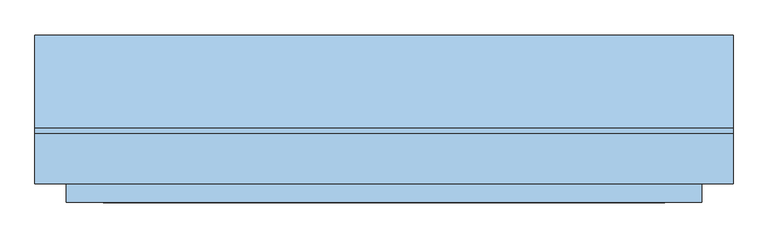
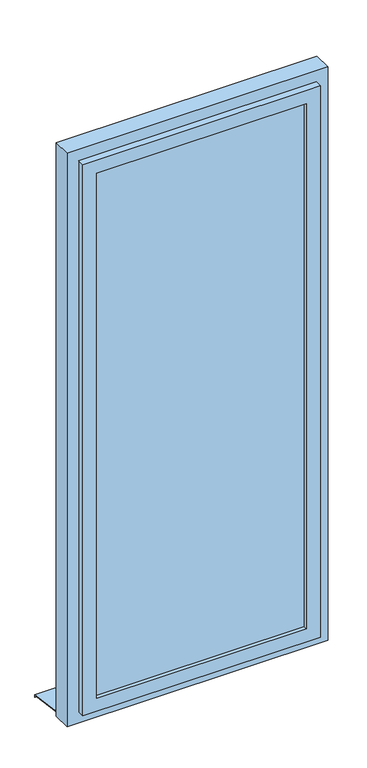
"""IFC4 building model written with IfcOpenShell, lengths in millimetres: window geometry, Fenstertür 1-flg : 1.80 x  3,1."""

from ifc_helpers import new_model, si_unit, frame, origin, place, context, project, spatial, polyline, outline, extrude, faceted_brep, source, transform, mapped, element, save


def window_6dc6708e(model_context):
    return source(origin(), model_context, "Body", "SolidModel", [
        extrude(outline(polyline([(2600.0, 560.0), (2600.0, -560.0), (0.0, -560.0), (0.0, 560.0), (2600.0, 560.0)]), holes=[polyline([(2520.0, 480.0), (80.0, 480.0), (80.0, -480.0), (2520.0, -480.0), (2520.0, 480.0)])]), frame((0.0, -58.6893832, 0.0), z_axis=(0.0, 1.0, 0.0), x_axis=(0.0, 0.0, 1.0)), (0.0, 0.0, 1.0), 80.0),
        faceted_brep([(510.0, -58.6893832, 2550.0), (510.0, -88.6893832, 2550.0), (510.0, -88.6893832, 50.0), (510.0, -58.6893832, 50.0), (-510.0, -88.6893832, 2550.0), (-510.0, -88.6893832, 50.0), (450.0, -88.6893832, 110.0), (-450.0, -88.6893832, 110.0), (-450.0, -88.6893832, 2490.0), (450.0, -88.6893832, 2490.0), (-510.0, -58.6893832, 50.0), (-510.0, -58.6893832, 2550.0), (480.0, -58.6893832, 2520.0), (-480.0, -58.6893832, 2520.0), (-480.0, -58.6893832, 80.0), (480.0, -58.6893832, 80.0), (480.0, -28.6893832, 2520.0), (480.0, -28.6893832, 80.0), (-480.0, -28.6893832, 80.0), (-480.0, -28.6893832, 2520.0), (450.0, -28.6893832, 2490.0), (-450.0, -28.6893832, 2490.0), (-450.0, -28.6893832, 110.0), (450.0, -28.6893832, 110.0)], [[[0, 1, 2, 3]], [[1, 4, 5, 2], [6, 7, 8, 9]], [[3, 2, 5, 10]], [[3, 10, 11, 0], [12, 13, 14, 15]], [[16, 12, 15, 17]], [[17, 15, 14, 18]], [[17, 18, 19, 16], [20, 21, 22, 23]], [[9, 20, 23, 6]], [[6, 23, 22, 7]], [[10, 5, 4, 11]], [[18, 14, 13, 19]], [[7, 22, 21, 8]], [[11, 4, 1, 0]], [[19, 13, 12, 16]], [[8, 21, 20, 9]]]),
        extrude(outline(polyline([(31.3327711, 20.0), (180.0, 0.0), (180.0, -10.0), (178.0, -10.0), (178.0, -1.6395366), (31.1346891, 18.0), (21.3106168, 18.0), (21.3106168, 20.0), (31.3327711, 20.0)])), frame((-560.0, 0.0, 0.0), z_axis=(1.0, 0.0, 0.0), x_axis=(0.0, 1.0, 0.0)), (0.0, 0.0, 1.0), 1120.0),
        extrude(outline(polyline([(450.0, -73.6893832), (-450.0, -73.6893832), (-450.0, -43.6893832), (450.0, -43.6893832), (450.0, -73.6893832)])), frame((0.0, 0.0, 110.0), z_axis=(0.0, 0.0, 1.0), x_axis=(1.0, 0.0, 0.0)), (0.0, 0.0, 1.0), 2380.0),
    ])


if __name__ == "__main__":
    model = new_model("IFC4")
    model_context = context("Model", 3, world=origin())
    ifc_project = project(units=[si_unit("LENGTHUNIT", "METRE", prefix="MILLI")], contexts=[model_context])
    site = spatial("IfcSite", under=ifc_project)
    building = spatial("IfcBuilding", under=site)
    placement = place(None, origin())
    window_shape = window_6dc6708e(model_context)
    element("IfcWindow", 1, ObjectType="Fenstertür 1-flg : 1.80 x  3,1", at=placement, inside=building, context=model_context, shape_type="MappedRepresentation", body=[
        mapped(window_shape, transform((0.0, 0.0, 0.0), x_axis=(1.0, 0.0, 0.0), y_axis=(0.0, 1.0, 0.0), z_axis=(0.0, 0.0, 1.0))),
    ])
    save(model, "model.ifc")

# Revit data of these elements
# Type "Fenstertür 1-flg : 1.80 x  3,1"
#   Type Mark = "51"
#   Operation = "SinglePanel"
#   Construction Type Id = "GSP4R"
#   Keynote = "16.05.01"
#   Analytic Construction = "1/8 Zoll Pilkington-Verglasung einfach"
#   Visual Light Transmittance = 0.9
#   Thermal Resistance (R) = 0.1491 (m²·K)/W
#   Solar Heat Gain Coefficient = 0.86
#   Rough Width = 1.120 m
#   Rough Height = 2.600 m
#   Heat Transfer Coefficient (U) = 6.7069 W/(m²·K)
#   Rahmentiefe = 0.080 m
#   Rahmenhöhe - unten = 0.080 m
#   Rahmenhöhe - oben = 0.080 m
#   Rahmenbreite = 0.080 m
#   Height = 2.600 m
#   Tiefe Flügel = 0.060 m
#   Flügelbreite = 0.060 m
#   Einbautiefe (von außen) [instance default] = 0.080 m
#   Width = 1.120 m
#   Kippflügel [instance default] = yes
#   Drehflügel im Grundriss darstellen [instance default] = yes
#   Drehflügel 1 [instance default] = yes
#   Rahmen 1 [instance default] = none
#   Glas [instance default] = none
#   Flügel [instance default] = none
#   Fensterbank Außenseite [instance default] = none
#   Wall Closure = (empty or 0)
# Element 1 (IfcWindow, "Fenstertür 1-flg : 1.80 x  3,1")
#   Einbautiefe (von außen) = 0.128689 m
#   Materials on its faces: "Kunststoff - Weiß", "Glas"
# Materials
#   "Kunststoff - Weiß": class "Kunststoff", colour RGB 249 249 249, transparency 0, Cost = 0
#   "Glas": class "Glas", colour RGB 0 0 255, transparency 0.75, Comments = "Render-Darstellung nicht aktualisiert ", Cost = 0
